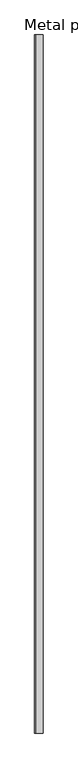
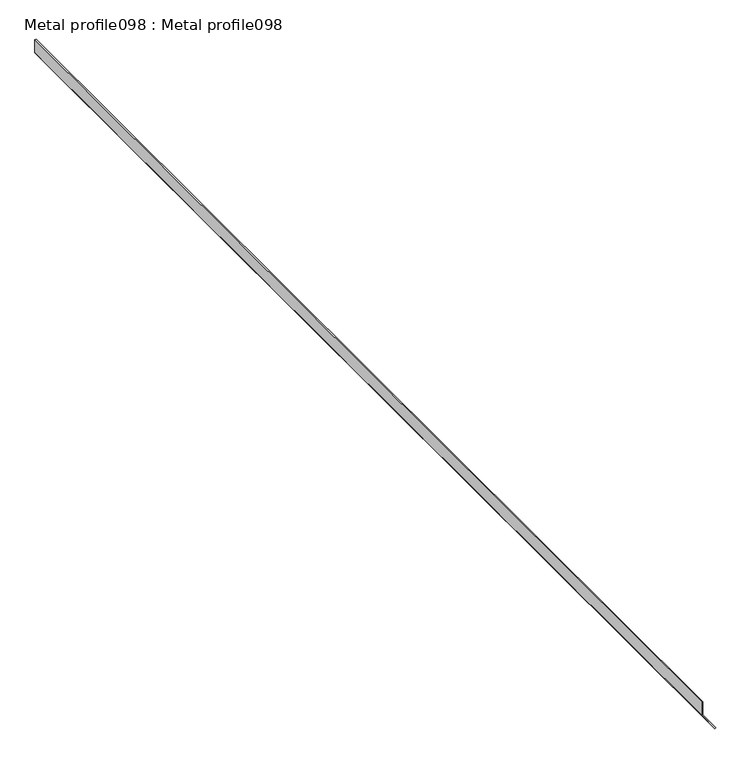
"""IFC4 building model written with IfcOpenShell, lengths in millimetres: proxy geometry, Metal profile098 : Metal profile098."""

from ifc_helpers import new_model, si_unit, frame, origin, place, context, project, spatial, polyline, outline, extrude, source, transform, mapped, element, save


def metal_profile098_metal_profile098_13732f97(model_context):
    return source(origin(), model_context, "Body", "SweptSolid", [
        extrude(outline(polyline([(43096.7438897, 17743.2484373), (43096.7438897, 17741.2484373), (43072.2907647, 17741.2484373), (43039.6306084, 17764.0926755), (43040.7769312, 17765.7315606), (43072.9208054, 17743.2484373), (43096.7438897, 17743.2484373)])), frame((0.0, 7982.1507711, 0.0), z_axis=(0.0, 1.0, 0.0), x_axis=(0.0, 0.0, 1.0)), (0.0, 0.0, 1.0), 2000.0),
    ])


if __name__ == "__main__":
    model = new_model("IFC4")
    model_context = context("Model", 3, world=origin())
    ifc_project = project(units=[si_unit("LENGTHUNIT", "METRE", prefix="MILLI")], contexts=[model_context])
    site = spatial("IfcSite", under=ifc_project)
    building = spatial("IfcBuilding", under=site)
    placement = place(None, origin())
    metal_profile098_metal_profile098_shape = metal_profile098_metal_profile098_13732f97(model_context)
    element("IfcBuildingElementProxy", 1, Name="Metal profile098 : Metal profile098", ObjectType="Metal profile098 : Metal profile098", at=placement, inside=building, context=model_context, shape_type="MappedRepresentation", body=[
        mapped(metal_profile098_metal_profile098_shape, transform((0.0, 0.0, 0.0), x_axis=(1.0, 0.0, 0.0), y_axis=(0.0, 1.0, 0.0), z_axis=(0.0, 0.0, 1.0))),
    ])
    save(model, "model.ifc")

# Revit data of these elements
# Type "Metal profile098 : Metal profile098"
#   NameOverride = "Metal profile098"
# Element 1 (IfcBuildingElementProxy, "Metal profile098 : Metal profile098")
#   Materials on its faces: "TRIM CLEAT"
# Materials
#   "TRIM CLEAT": class "Unassigned", colour RGB 255 232 5, transparency 0
